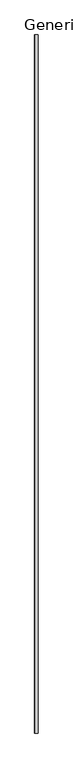
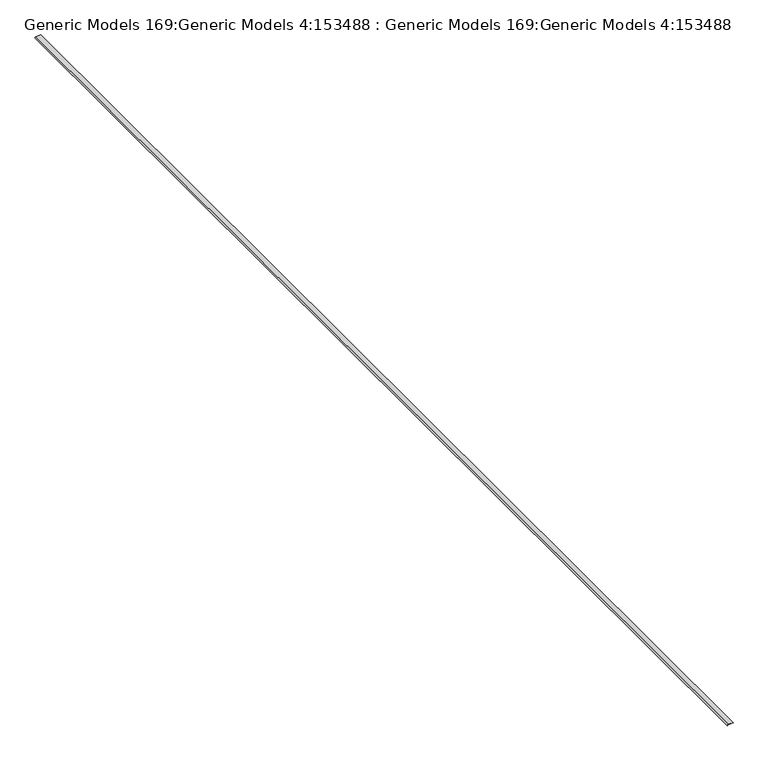
"""IFC4 building model written with IfcOpenShell, lengths in millimetres: proxy geometry, Generic Models 169:Generic Models 4:153488 : Generic Models 169:Generic Models 4:153488."""

from ifc_helpers import new_model, si_unit, frame, origin, place, context, project, spatial, polyline, outline, extrude, source, transform, mapped, element, save


def generic_models_169_generic_models_4_153488_generic_models_cb98e6ea(model_context):
    return source(origin(), model_context, "Body", "SweptSolid", [
        extrude(outline(polyline([(-360.8398941, -10339.4822511), (-350.4366632, -10332.1978304), (-350.4366632, -10279.9172058), (-348.8491632, -10279.9172058), (-348.8491632, -10333.0242306), (-359.9293415, -10340.782655), (-360.8398941, -10339.4822511)])), frame((0.0, -5303.1974793, 0.0), z_axis=(0.0, 1.0, 0.0), x_axis=(0.0, 0.0, 1.0)), (0.0, 0.0, 1.0), 12547.6),
    ])


if __name__ == "__main__":
    model = new_model("IFC4")
    model_context = context("Model", 3, world=origin())
    ifc_project = project(units=[si_unit("LENGTHUNIT", "METRE", prefix="MILLI")], contexts=[model_context])
    site = spatial("IfcSite", under=ifc_project)
    building = spatial("IfcBuilding", under=site)
    placement = place(None, origin())
    generic_models_169_generic_models_4_153488_generic_models_shape = generic_models_169_generic_models_4_153488_generic_models_cb98e6ea(model_context)
    element("IfcBuildingElementProxy", 1, Name="Generic Models 169:Generic Models 4:153488 : Generic Models 169:Generic Models 4:153488", ObjectType="Generic Models 169:Generic Models 4:153488 : Generic Models 169:Generic Models 4:153488", at=placement, inside=building, context=model_context, shape_type="MappedRepresentation", body=[
        mapped(generic_models_169_generic_models_4_153488_generic_models_shape, transform((0.0, 0.0, 0.0), x_axis=(1.0, 0.0, 0.0), y_axis=(0.0, 1.0, 0.0), z_axis=(0.0, 0.0, 1.0))),
    ])
    save(model, "model.ifc")

# Revit data of these elements
# Type "Generic Models 169:Generic Models 4:153488 : Generic Models 169:Generic Models 4:153488"
#   NameOverride = "Generic Models 169:Generic Models 4:153488"
#   ObjectTypeOverride = "Generic Models 169:Generic Models 4"
#   Reference = "Generic Models 4"
#   Category = "Generic Models"
#   Tag = "153488"
# Element 1 (IfcBuildingElementProxy, "Generic Models 169:Generic Models 4:153488 : Generic Models 169:Generic Models 4:153488")
#   Materials on its faces: "_CONT. 16 GA. COPPER DRIP FLASHING"
# Materials
#   "_CONT. 16 GA. COPPER DRIP FLASHING": class "Metal", colour RGB 199 199 199, transparency 0, Description = "Structural steel 50ksi", Cost = 0
